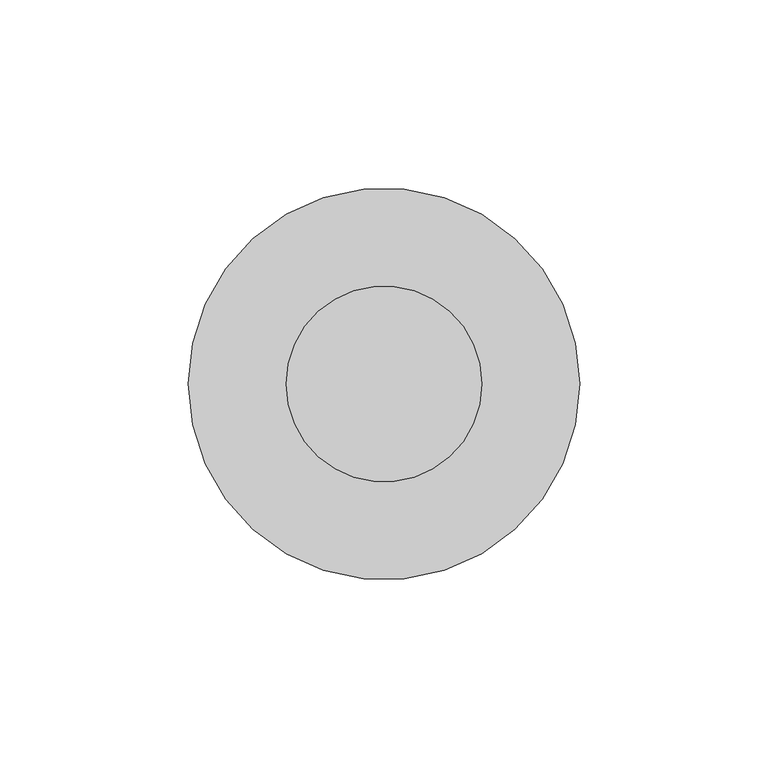
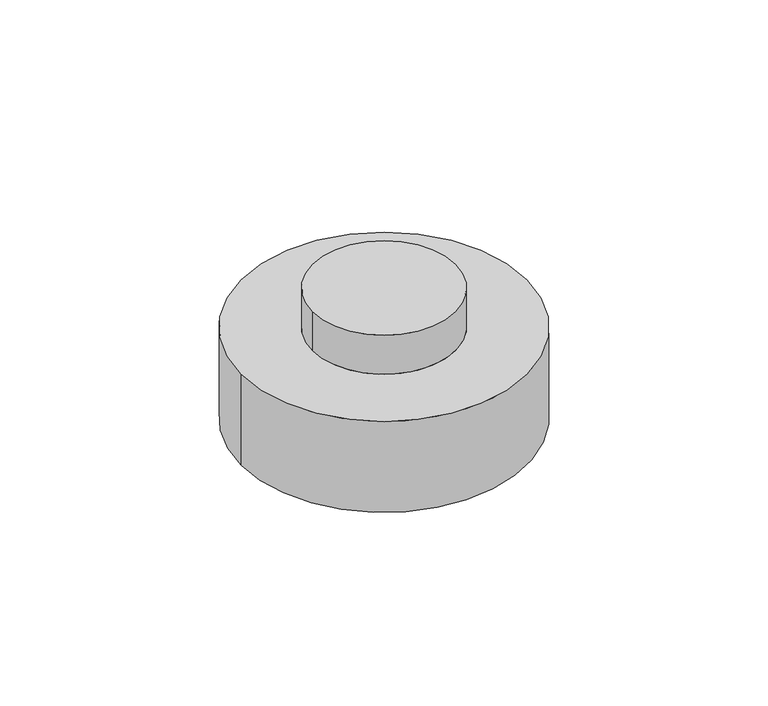
"""IFC4 building model written with IfcOpenShell, lengths in millimetres: alarm geometry, 光电感烟探测器 : 点型."""

from ifc_helpers import new_model, si_unit, frame, origin, origin_with_axes, place, context, project, spatial, circle_curve, source, transform, mapped, element, save
from ifc_brep_helpers import plane_surface, cylinder_surface, advanced_brep


def alarm_5285ee31(model_context):
    return source(origin(), model_context, "Body", "AdvancedBrep", [
        advanced_brep(
        [(-26.0, 0.0, 50.0), (26.0, 0.0, 50.0), (-52.0, 0.0, 0.0), (52.0, 0.0, 0.0), (-26.0, 0.0, 35.0), (26.0, 0.0, 35.0), (-52.0, 0.0, 35.0), (52.0, 0.0, 35.0)],
        [
            (0, 1, circle_curve(frame((0.0, 0.0, 50.0), z_axis=(0.0, 0.0, 1.0), x_axis=(1.0, 0.0, 0.0)), 26.0)),
            (1, 0, circle_curve(frame((0.0, 0.0, 50.0), z_axis=(0.0, 0.0, 1.0), x_axis=(1.0, 0.0, 0.0)), 26.0)),
            (2, 3, circle_curve(frame((0.0, 0.0, 0.0), z_axis=(0.0, 0.0, -1.0), x_axis=(1.0, 0.0, 0.0)), 52.0)),
            (3, 2, circle_curve(frame((0.0, 0.0, 0.0), z_axis=(0.0, 0.0, -1.0), x_axis=(1.0, 0.0, 0.0)), 52.0)),
            (0, 4),
            (4, 5, circle_curve(frame((0.0, 0.0, 35.0), z_axis=(0.0, 0.0, 1.0), x_axis=(1.0, 0.0, 0.0)), 26.0)),
            (5, 1),
            (5, 4, circle_curve(frame((0.0, 0.0, 35.0), z_axis=(0.0, 0.0, 1.0), x_axis=(1.0, 0.0, 0.0)), 26.0)),
            (6, 7, circle_curve(frame((0.0, 0.0, 35.0), z_axis=(0.0, 0.0, 1.0), x_axis=(1.0, 0.0, 0.0)), 52.0)),
            (7, 6, circle_curve(frame((0.0, 0.0, 35.0), z_axis=(0.0, 0.0, 1.0), x_axis=(1.0, 0.0, 0.0)), 52.0)),
            (3, 7),
            (6, 2),
        ],
        [
            plane_surface(frame((26.0, 0.0, 50.0), z_axis=(0.0, 0.0, 1.0), x_axis=(0.0, 1.0, 0.0))),
            plane_surface(frame((26.0, 0.0, 0.0), z_axis=(0.0, 0.0, -1.0), x_axis=(0.0, -1.0, 0.0))),
            cylinder_surface(origin_with_axes(), 26.0),
            plane_surface(frame((52.0, 0.0, 35.0), z_axis=(0.0, 0.0, 1.0), x_axis=(0.0, 1.0, 0.0))),
            cylinder_surface(origin_with_axes(), 52.0),
        ],
        [
            (0, [[1, 2]]),
            (1, [[3, 4]]),
            (2, [[-1, 5, 6, 7]]),
            (2, [[-2, -7, 8, -5]]),
            (3, [[9, 10], [-6, -8]]),
            (4, [[-4, 11, -9, 12]]),
            (4, [[-3, -12, -10, -11]]),
        ],
    ),
    ])


if __name__ == "__main__":
    model = new_model("IFC4")
    model_context = context("Model", 3, world=origin())
    ifc_project = project(units=[si_unit("LENGTHUNIT", "METRE", prefix="MILLI")], contexts=[model_context])
    site = spatial("IfcSite", under=ifc_project)
    building = spatial("IfcBuilding", under=site)
    placement = place(None, origin())
    alarm_shape = alarm_5285ee31(model_context)
    element("IfcAlarm", 1, ObjectType="光电感烟探测器 : 点型", at=placement, inside=building, context=model_context, shape_type="MappedRepresentation", body=[
        mapped(alarm_shape, transform((0.0, 0.0, 0.0), x_axis=(1.0, 0.0, 0.0), y_axis=(0.0, 1.0, 0.0), z_axis=(0.0, 0.0, 1.0))),
    ])
    save(model, "model.ifc")

# Revit data of these elements
# Type "光电感烟探测器 : 点型"
#   半径 3 = 36.77 mm
#   半径 2 = 52 mm
#   半径 1 = 26 mm
#   高度 2 = 15 mm
#   高度 1 = 35 mm
#   Default Elevation = 1200 mm
#   可见性 2 = no
#   可见性 1 = yes
#   材质 = none
